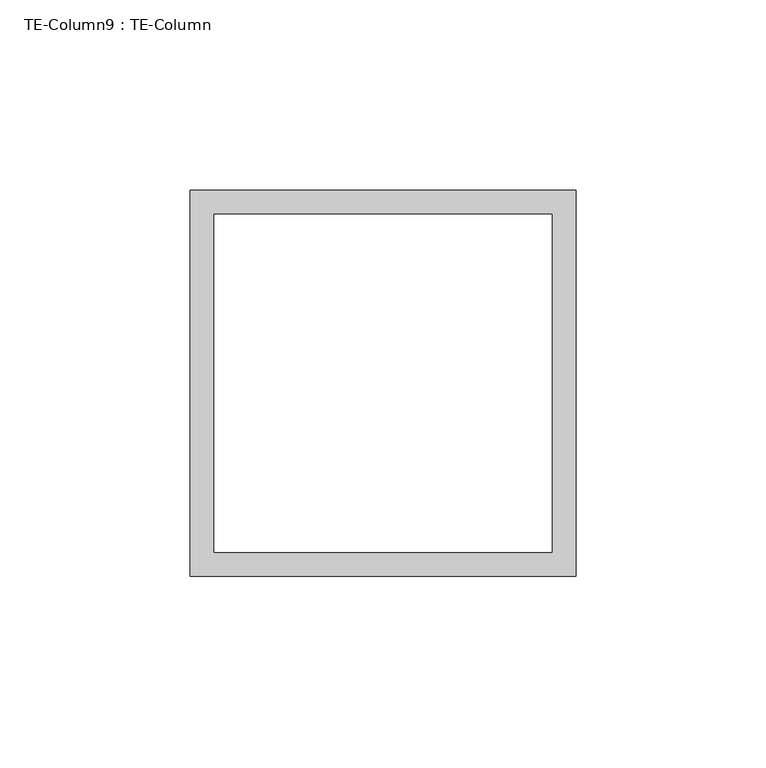
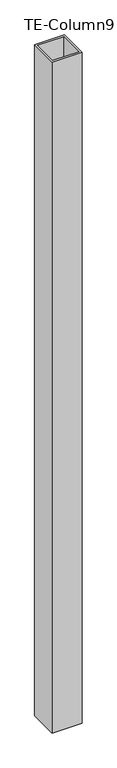
"""IFC4 building model written with IfcOpenShell, lengths in millimetres: proxy geometry, TE-Column9 : TE-Column."""

from ifc_helpers import new_model, si_unit, frame, origin, place, context, project, spatial, polyline, outline, extrude, source, transform, mapped, element, save


def te_column9_te_column_de7abfcb(model_context):
    return source(origin(), model_context, "Body", "SweptSolid", [
        extrude(outline(polyline([(588893.0684739, -531667.7913841), (588893.0684739, -531769.3913841), (588791.4684739, -531769.3913841), (588791.4684739, -531667.7913841), (588893.0684739, -531667.7913841)]), holes=[polyline([(588797.8184739, -531674.1413841), (588797.8184739, -531763.0413841), (588886.7184739, -531763.0413841), (588886.7184739, -531674.1413841), (588797.8184739, -531674.1413841)])]), frame((0.0, 0.0, 28.575), z_axis=(0.0, 0.0, 1.0), x_axis=(1.0, 0.0, 0.0)), (0.0, 0.0, 1.0), 2406.65),
    ])


if __name__ == "__main__":
    model = new_model("IFC4")
    model_context = context("Model", 3, world=origin())
    ifc_project = project(units=[si_unit("LENGTHUNIT", "METRE", prefix="MILLI")], contexts=[model_context])
    site = spatial("IfcSite", under=ifc_project)
    building = spatial("IfcBuilding", under=site)
    placement = place(None, origin())
    te_column9_te_column_shape = te_column9_te_column_de7abfcb(model_context)
    element("IfcBuildingElementProxy", 1, Name="TE-Column9 : TE-Column", ObjectType="TE-Column9 : TE-Column", at=placement, inside=building, context=model_context, shape_type="MappedRepresentation", body=[
        mapped(te_column9_te_column_shape, transform((0.0, 0.0, 0.0), x_axis=(1.0, 0.0, 0.0), y_axis=(0.0, 1.0, 0.0), z_axis=(0.0, 0.0, 1.0))),
    ])
    save(model, "model.ifc")

# Revit data of these elements
# Element 1 (IfcBuildingElementProxy, "TE-Column9 : TE-Column")
#   Materials on its faces: "4\"X4\" GALV. HSS TUBING"
# Materials
#   "4\"X4\" GALV. HSS TUBING": class "Generic", colour RGB 211 211 207, transparency 0, Cost = 0
